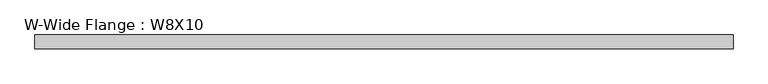
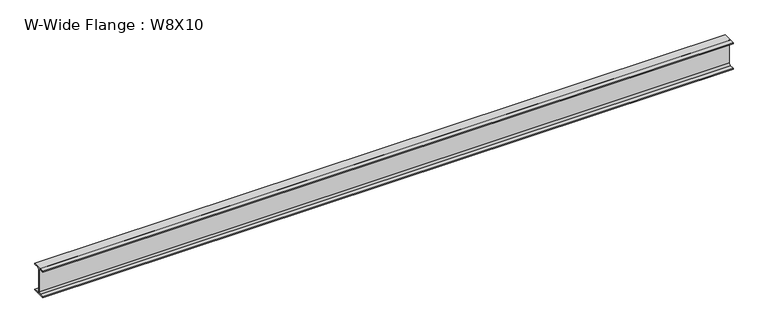
"""IFC4 building model written with IfcOpenShell, lengths in millimetres: beam geometry, W-Wide Flange : W8X10."""

from ifc_helpers import new_model, si_unit, point, frame, frame_2d, origin, place, context, project, spatial, polyline, circle_curve, trimmed, segment, composite_curve, outline, extrude, source, transform, mapped, element, save


def w_wide_flange_w8x10_4803d970(model_context):
    return source(origin(), model_context, "Body", "SweptSolid", [
        extrude(outline(composite_curve([segment(polyline([(50.038, -94.996), (50.038, -100.203), (-50.038, -100.203), (-50.038, -94.996), (-14.4145, -94.996)]), True, "CONTINUOUS"), segment(trimmed(circle_curve(frame_2d((-14.4145, -82.7405)), 12.2555), [point((-14.4145, -94.996))], [point((-2.159, -82.7405))], True, "CARTESIAN"), True, "CONTINUOUS"), segment(polyline([(-2.159, -82.7405), (-2.159, 82.7405)]), True, "CONTINUOUS"), segment(trimmed(circle_curve(frame_2d((-14.4145, 82.7405)), 12.2555), [point((-2.159, 82.7405))], [point((-14.4145, 94.996))], True, "CARTESIAN"), True, "CONTINUOUS"), segment(polyline([(-14.4145, 94.996), (-50.038, 94.996), (-50.038, 100.203), (50.038, 100.203), (50.038, 94.996), (14.4145, 94.996)]), True, "CONTINUOUS"), segment(trimmed(circle_curve(frame_2d((14.4145, 82.7405)), 12.2555), [point((14.4145, 94.996))], [point((2.159, 82.7405))], True, "CARTESIAN"), True, "CONTINUOUS"), segment(polyline([(2.159, 82.7405), (2.159, -82.7405)]), True, "CONTINUOUS"), segment(trimmed(circle_curve(frame_2d((14.4145, -82.7405)), 12.2555), [point((2.159, -82.7405))], [point((14.4145, -94.996))], True, "CARTESIAN"), True, "CONTINUOUS"), segment(polyline([(14.4145, -94.996), (50.038, -94.996)]), True, "CONTINUOUS")], self_intersect=False)), frame((-2487.0171875, 0.0, 0.0), z_axis=(1.0, 0.0, 0.0), x_axis=(0.0, 1.0, 0.0)), (0.0, 0.0, 1.0), 4990.5046875),
    ])


if __name__ == "__main__":
    model = new_model("IFC4")
    model_context = context("Model", 3, world=origin())
    ifc_project = project(units=[si_unit("LENGTHUNIT", "METRE", prefix="MILLI")], contexts=[model_context])
    site = spatial("IfcSite", under=ifc_project)
    building = spatial("IfcBuilding", under=site)
    placement = place(None, origin())
    w_wide_flange_w8x10_shape = w_wide_flange_w8x10_4803d970(model_context)
    element("IfcBeam", 1, ObjectType="W-Wide Flange : W8X10", at=placement, inside=building, context=model_context, shape_type="MappedRepresentation", body=[
        mapped(w_wide_flange_w8x10_shape, transform((0.0, 0.0, 0.0), x_axis=(1.0, 0.0, 0.0), y_axis=(0.0, 1.0, 0.0), z_axis=(0.0, 0.0, 1.0))),
    ])
    save(model, "model.ifc")

# Revit data of these elements
# Type "W-Wide Flange : W8X10"
#   Assembly Code = "B10"
#   W = 10
#   Length [instance default] = 1524 mm
#   bf = 100.076 mm
#   d = 200.406 mm
#   k = 17.463 mm
#   k2 = 12.255 mm
#   tf = 5.207 mm
#   tw = 4.318 mm
#   A = 0.00190967 m²
#   Structural Material [instance default] = Steel ASTM A992
# Element 1 (IfcBeam, "W-Wide Flange : W8X10")
#   Structural Material = Aluminum, Anodized Red
#   Materials on its faces: "Aluminum, Anodized Red"
# Materials
#   "Steel ASTM A992": class "Metal", colour RGB 128 0 0, transparency 0, Description = "Structural steel 50ksi", Cost = 0
#   "Aluminum, Anodized Red": class "Metal", colour RGB 120 120 120, transparency 0, Description = "Anodized aluminum, red", Cost = 0
